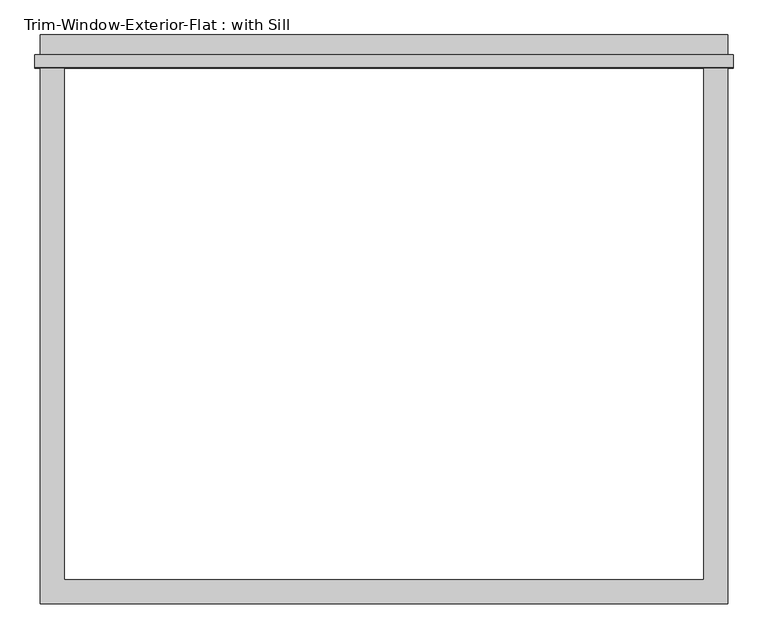
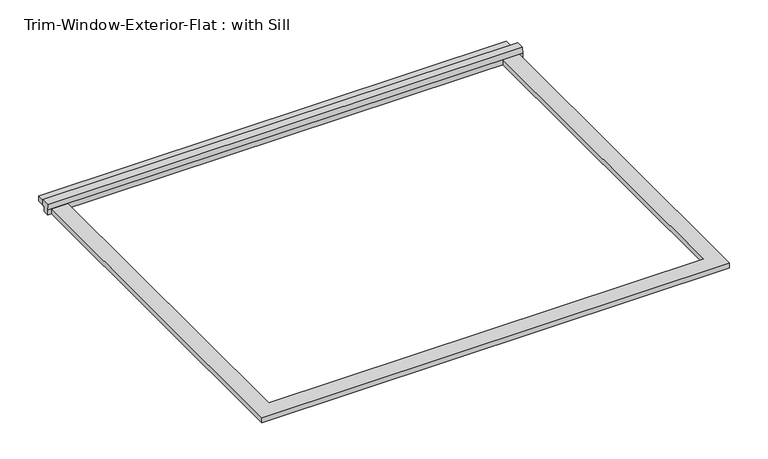
"""IFC4 building model written with IfcOpenShell, lengths in millimetres: proxy geometry, Trim-Window-Exterior-Flat : with Sill."""

import ifcopenshell
import ifcopenshell.guid

model = None  # the IFC model being written
_history = None  # IfcOwnerHistory: only IFC2X3 demands one
_inside = {}  # id of a spatial element -> (the spatial element, [elements in it])
_under = {}  # id of a project, library or spatial element -> (it, [spatial elements below it])
_declared = {}  # id of a project -> (the project, [libraries it declares])
_typed = {}  # id of a type object -> (the type object, [elements of that type])
_made_of = {}  # id of a material, layer set ... -> (it, [elements and type objects made of it])


def new_model(schema):
    """Start an empty IFC model of exactly this schema.

    Asked for "IFC4X3", IfcOpenShell would pick the latest addendum, in which some entities
    have other attributes; the version numbers below select the first issue.
    IFC2X3 requires an IfcOwnerHistory on every rooted entity: one is made here for all.
    """
    global model, _history
    if schema == "IFC4X3":
        model = ifcopenshell.file(schema_version=(4, 3, 0, 0))
    else:
        model = ifcopenshell.file(schema=schema)
    _inside.clear()
    _under.clear()
    _declared.clear()
    _typed.clear()
    _made_of.clear()
    _history = None
    if model.schema == "IFC2X3":
        org = make("IfcOrganization", Name="unknown")
        user = make(
            "IfcPersonAndOrganization",
            ThePerson=make("IfcPerson", FamilyName="unknown"),
            TheOrganization=org,
        )
        app = make(
            "IfcApplication",
            ApplicationDeveloper=org,
            Version="unknown",
            ApplicationFullName="unknown",
            ApplicationIdentifier="unknown",
        )
        _history = make(
            "IfcOwnerHistory",
            OwningUser=user,
            OwningApplication=app,
            ChangeAction="ADDED",
            CreationDate=0,
        )
    return model


def make(cls, **values):
    """One entity of the class cls with the attributes given. An attribute that is None is left unset."""
    return model.create_entity(
        cls, **{name: value for name, value in values.items() if value is not None}
    )


def rooted(cls, **values):
    """An entity with a GlobalId (a new one), such as an element, a storey or a relation."""
    return make(cls, GlobalId=ifcopenshell.guid.new(), OwnerHistory=_history, **values)


def si_unit(unit_type, name, prefix=None):
    """IfcSIUnit, for example si_unit("LENGTHUNIT", "METRE", prefix="MILLI")."""
    return make("IfcSIUnit", UnitType=unit_type, Prefix=prefix, Name=name)


def assignment(units):
    """IfcUnitAssignment: the units of a project."""
    return None if units is None else make("IfcUnitAssignment", Units=units)


def point(xyz):
    """IfcCartesianPoint."""
    return None if xyz is None else make("IfcCartesianPoint", Coordinates=xyz)


def direction(xyz):
    """IfcDirection."""
    return None if xyz is None else make("IfcDirection", DirectionRatios=xyz)


def frame(location, z_axis=None, x_axis=None):
    """IfcAxis2Placement3D, a coordinate frame: its origin and axes. An axis left out is left unset."""
    return make(
        "IfcAxis2Placement3D",
        Location=point(location),
        Axis=direction(z_axis),
        RefDirection=direction(x_axis),
    )


def origin():
    """The frame at (0, 0, 0) with its axes left unset."""
    return frame((0.0, 0.0, 0.0))


def origin_with_axes():
    """The frame at (0, 0, 0) with the z axis (0, 0, 1) and the x axis (1, 0, 0) written out."""
    return frame((0.0, 0.0, 0.0), z_axis=(0.0, 0.0, 1.0), x_axis=(1.0, 0.0, 0.0))


def place(relative_to, where):
    """IfcLocalPlacement: puts the frame where relative to a parent placement (None: the world)."""
    return make(
        "IfcLocalPlacement", PlacementRelTo=relative_to, RelativePlacement=where
    )


def context(
    kind, dimensions, precision=None, world=None, true_north=None, identifier=None
):
    """IfcGeometricRepresentationContext, for example the 3D "Model" context."""
    return make(
        "IfcGeometricRepresentationContext",
        ContextIdentifier=identifier,
        ContextType=kind,
        CoordinateSpaceDimension=dimensions,
        Precision=precision,
        WorldCoordinateSystem=world,
        TrueNorth=true_north,
    )


def project(units=None, contexts=None):
    """IfcProject with its units and contexts."""
    return rooted(
        "IfcProject",
        Name="project",
        RepresentationContexts=contexts,
        UnitsInContext=assignment(units),
    )


def spatial(cls, under=None, at=None, **own):
    """A site, building, storey or space (cls), placed at a placement, below another one or the project."""
    s = rooted(cls, ObjectPlacement=at, **own)
    if under is not None:
        _under.setdefault(under.id(), (under, []))[1].append(s)
    return s


def polyline(points):
    """IfcPolyline through the points."""
    return make("IfcPolyline", Points=[point(p) for p in points])


def outline(outer, holes=None, kind="AREA"):
    """IfcArbitraryClosedProfileDef: a profile drawn as a closed curve; with holes, ...WithVoids."""
    if holes is None:
        return make("IfcArbitraryClosedProfileDef", ProfileType=kind, OuterCurve=outer)
    return make(
        "IfcArbitraryProfileDefWithVoids",
        ProfileType=kind,
        OuterCurve=outer,
        InnerCurves=holes,
    )


def extrude(swept, where, along, depth):
    """IfcExtrudedAreaSolid: the profile swept, set in the frame where, extruded along a direction by depth."""
    return make(
        "IfcExtrudedAreaSolid",
        SweptArea=swept,
        Position=where,
        ExtrudedDirection=direction(along),
        Depth=depth,
    )


def shape(context_of_items, identifier, shape_type, items):
    """IfcShapeRepresentation: the items that make up one representation, for example the "Body"."""
    return make(
        "IfcShapeRepresentation",
        ContextOfItems=context_of_items,
        RepresentationIdentifier=identifier,
        RepresentationType=shape_type,
        Items=items,
    )


def source(mapping_origin, context_of_items, identifier, shape_type, items):
    """IfcRepresentationMap: a shape defined once, which mapped items show again and again."""
    return make(
        "IfcRepresentationMap",
        MappingOrigin=mapping_origin,
        MappedRepresentation=shape(context_of_items, identifier, shape_type, items),
    )


def transform(
    local_origin,
    x_axis=None,
    y_axis=None,
    z_axis=None,
    scale=None,
    scale2=None,
    scale3=None,
    uniform=True,
):
    """IfcCartesianTransformationOperator3D, or its non-uniform kind. x_axis, y_axis, z_axis: its Axis1, 2, 3."""
    if uniform:
        return make(
            "IfcCartesianTransformationOperator3D",
            Axis1=direction(x_axis),
            Axis2=direction(y_axis),
            LocalOrigin=point(local_origin),
            Scale=scale,
            Axis3=direction(z_axis),
        )
    return make(
        "IfcCartesianTransformationOperator3DnonUniform",
        Axis1=direction(x_axis),
        Axis2=direction(y_axis),
        LocalOrigin=point(local_origin),
        Scale=scale,
        Axis3=direction(z_axis),
        Scale2=scale2,
        Scale3=scale3,
    )


def mapped(mapping_source, mapping_target):
    """IfcMappedItem: shows the shape of a source again, moved by a transform."""
    return make(
        "IfcMappedItem", MappingSource=mapping_source, MappingTarget=mapping_target
    )


def made_of(thing, what):
    """Note that an element or type object is made of a material, layer set ...; save() writes the relation."""
    if what is not None:
        _made_of.setdefault(what.id(), (what, []))[1].append(thing)
    return thing


def element(
    cls,
    number,
    at=None,
    inside=None,
    cuts=None,
    type_object=None,
    material=None,
    context=None,
    identifier="Body",
    shape_type=None,
    held_by="IfcProductDefinitionShape",
    body=None,
    shapes=None,
    **own,
):
    """One element of the class cls, such as IfcWall. Its Tag is "e" and its number.

    at: its placement. inside: the storey or other place that contains it. cuts: it is an
    opening in that element (IfcRelVoidsElement). A single representation is given by context,
    identifier, shape_type and body (its items); several are given by shapes. held_by: the class
    of the entity that holds the representations. save() writes the other relations.
    """
    e = rooted(cls, Tag="e%d" % number, ObjectPlacement=at, **own)
    if body is not None:
        shapes = [shape(context, identifier, shape_type, body)]
    if shapes is not None:
        e.Representation = make(held_by, Representations=shapes)
    if inside is not None:
        _inside.setdefault(inside.id(), (inside, []))[1].append(e)
    if cuts is not None:
        rooted(
            "IfcRelVoidsElement", RelatingBuildingElement=cuts, RelatedOpeningElement=e
        )
    if type_object is not None:
        _typed.setdefault(type_object.id(), (type_object, []))[1].append(e)
    return made_of(e, material)


def aggregate(whole, parts):
    """IfcRelAggregates: a whole, such as a stair, and the parts it consists of."""
    return rooted("IfcRelAggregates", RelatingObject=whole, RelatedObjects=parts)


def save(model, path):
    """Write the relations noted so far, then the file.

    IfcRelAggregates (storeys below a building ...), IfcRelContainedInSpatialStructure (elements
    in a storey), IfcRelDefinesByType, IfcRelAssociatesMaterial and IfcRelDeclares: one each for
    every whole, place, type object, material and project.
    """
    for whole, parts in _under.values():
        aggregate(whole, parts)
    for where, things in _inside.values():
        rooted(
            "IfcRelContainedInSpatialStructure",
            RelatedElements=things,
            RelatingStructure=where,
        )
    for kind, things in _typed.values():
        rooted("IfcRelDefinesByType", RelatedObjects=things, RelatingType=kind)
    for what, things in _made_of.values():
        rooted("IfcRelAssociatesMaterial", RelatedObjects=things, RelatingMaterial=what)
    for by, libraries in _declared.values():
        rooted("IfcRelDeclares", RelatingContext=by, RelatedDefinitions=libraries)
    model.write(path)


def trim_window_exterior_flat_with_sill_59c7181e(model_context):
    return source(origin(), model_context, "Body", "SweptSolid", [
        extrude(outline(polyline([(819.15, 1241.3823709), (-819.15, 1241.3823709), (-819.15, 1298.5323709), (819.15, 1298.5323709), (819.15, 1241.3823709)])), origin_with_axes(), (0.0, 0.0, 1.0), 19.05),
        extrude(outline(polyline([(1250.95, 38.1), (1250.95, 19.05), (1241.3823709, 19.05), (1241.3823709, 0.0), (1219.2, 0.0), (1219.2, 19.05), (1221.6580645, 38.1), (1250.95, 38.1)])), frame((-831.85, 0.0, 0.0), z_axis=(1.0, 0.0, 0.0), x_axis=(0.0, 1.0, 0.0)), (0.0, 0.0, 1.0), 1663.7),
        extrude(outline(polyline([(-819.15, -57.15), (-819.15, 1219.2), (-762.0, 1219.2), (-762.0, 0.0), (762.0, 0.0), (762.0, 1219.2), (819.15, 1219.2), (819.15, -57.15), (-819.15, -57.15)])), origin_with_axes(), (0.0, 0.0, 1.0), 19.05),
    ])


if __name__ == "__main__":
    model = new_model("IFC4")
    model_context = context("Model", 3, world=origin())
    ifc_project = project(units=[si_unit("LENGTHUNIT", "METRE", prefix="MILLI")], contexts=[model_context])
    site = spatial("IfcSite", under=ifc_project)
    building = spatial("IfcBuilding", under=site)
    placement = place(None, origin())
    trim_window_exterior_flat_with_sill_shape = trim_window_exterior_flat_with_sill_59c7181e(model_context)
    element("IfcBuildingElementProxy", 1, Name="Trim-Window-Exterior-Flat : with Sill", ObjectType="Trim-Window-Exterior-Flat : with Sill", at=placement, inside=building, context=model_context, shape_type="MappedRepresentation", body=[
        mapped(trim_window_exterior_flat_with_sill_shape, transform((0.0, 0.0, 0.0), x_axis=(1.0, 0.0, 0.0), y_axis=(0.0, 1.0, 0.0), z_axis=(0.0, 0.0, 1.0))),
    ])
    save(model, "model.ifc")

# Revit data of these elements
# Type "Trim-Window-Exterior-Flat : with Sill"
#   Trim Width = 0' - 2 1/4"
#   Trim Thickness_Picture Frame = 0' - 1 1/4"
#   Trim Thickness_with Sill = 0' - 0 3/4"
#   Sill Thickness = 0' - 1 1/4"
#   Opening Width [instance default] = 2' - 0"
#   Opening Height [instance default] = 3' - 0"
#   Default Elevation = 4' - 0"
#   Sill = yes
#   Picture Frame = no
#   Trim Material [instance default] = none
# Element 1 (IfcBuildingElementProxy, "Trim-Window-Exterior-Flat : with Sill")
#   Opening Width = 5' - 0"
#   Opening Height = 4' - 0"
#   Trim Material = PVC, Flexible
#   Materials on its faces: "PVC, Flexible"
# Materials
#   "PVC, Flexible": class "Plastic", colour RGB 178 178 178, transparency 0, Description = "Flexible polyvinyl chloride", Cost = 0
